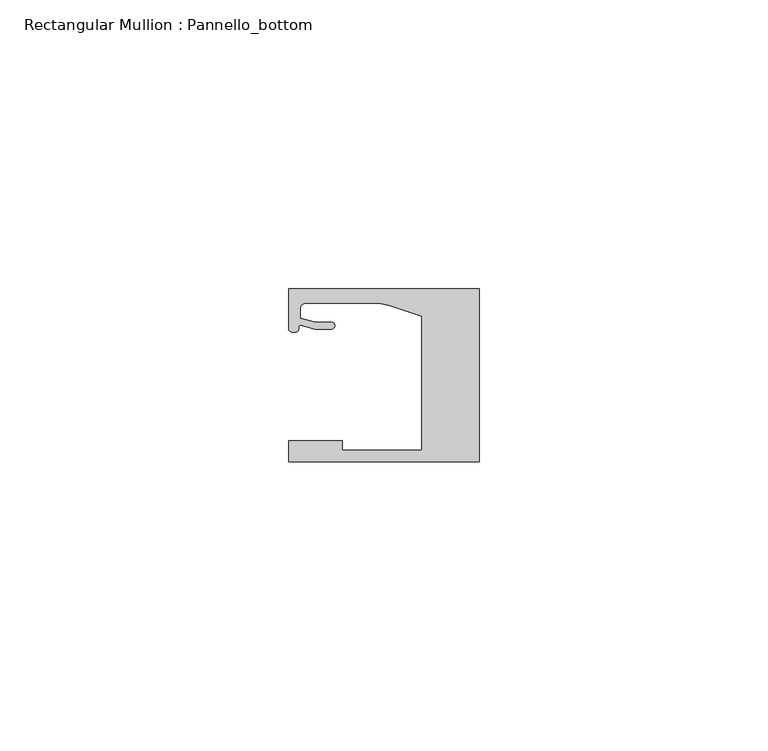
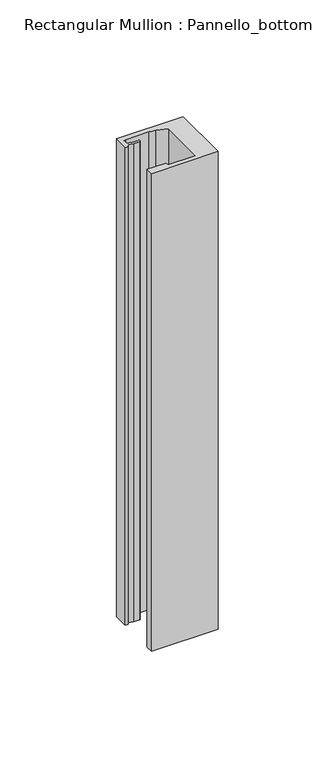
"""IFC4 building model written with IfcOpenShell, lengths in millimetres: member geometry, Rectangular Mullion : Pannello_bottom."""

from ifc_helpers import new_model, si_unit, frame, origin, place, context, project, spatial, polyline, circle_curve, source, transform, mapped, element, save
from ifc_brep_helpers import plane_surface, cylinder_surface, revolved_surface, extruded_surface, spline_curve, advanced_brep


def rectangular_mullion_pannello_bottom_a739c707(model_context):
    return source(origin(), model_context, "Body", "AdvancedBrep", [
        advanced_brep(
        [(-33.0, -15.0, 0.0), (0.0, -15.0, 0.0), (0.0, 15.0, 0.0), (-33.0000135, 15.0, 0.0), (-33.0000135, 8.0000472, 0.0), (-30.9223017, 8.6490241, 0.0), (-28.4999305, 7.9999523, 0.0), (-25.59998, 7.9999523, 0.0), (-25.59998, 9.1999523, 0.0), (-28.3419477, 9.1999523, 0.0), (-31.0, 9.9121746, 0.0), (-31.0, 11.4999419, 0.0), (-30.0000002, 12.4999419, 0.0), (-18.5493024, 12.4999438, 0.0), (-15.4591336, 12.0105099, 0.0), (-9.9999723, 10.2367227, 0.0), (-9.9999723, -13.0000004, 0.0), (-23.700041, -13.0000004, 0.0), (-23.700041, -11.3000004, 0.0), (-33.0, -11.3000004, 0.0), (-33.0, -15.0, -250.0), (-33.0, -11.3000004, -250.0), (-23.700041, -11.3000004, -250.0), (-23.700041, -13.0000004, -250.0), (-9.9999723, -13.0000004, -250.0), (-9.9999723, 10.2367227, -250.0), (-15.4591336, 12.0105099, -250.0), (-18.5493024, 12.4999438, -250.0), (-30.0000002, 12.4999419, -250.0), (-31.0, 11.4999419, -250.0), (-31.0, 9.9121746, -250.0), (-28.3419477, 9.1999523, -250.0), (-25.59998, 9.1999523, -250.0), (-25.59998, 7.9999523, -250.0), (-28.4999305, 7.9999523, -250.0), (-30.9223017, 8.6490241, -250.0), (-33.0000135, 8.0000472, -250.0), (-33.0000135, 15.0, -250.0), (0.0, 15.0, -250.0), (0.0, -15.0, -250.0)],
        [
            (0, 1),
            (1, 2),
            (2, 3),
            (3, 4),
            (4, 5, spline_curve(3, [(-33.0000135, 8.0000472, 0.0), (-33.0000135, 7.457047519, 0.0), (-32.262327879, 7.456527435, 0.0), (-31.357433266, 7.563996614, 0.0), (-31.305645054, 7.690065204, 0.0), (-31.298563602, 8.366228555, 0.0), (-31.312054066, 8.717747958, 0.0), (-30.9223017, 8.6490241, 0.0)], [4, 2, 2, 4], [0.0, 0.0027053965905959043, 0.0058611956533709, 0.007702013405570312])),
            (5, 6),
            (6, 7),
            (7, 8, circle_curve(frame((-25.59998, 8.5999523, 0.0), z_axis=(0.0, 0.0, 1.0), x_axis=(0.0, 1.0, 0.0)), 0.6)),
            (8, 9),
            (9, 10),
            (10, 11),
            (11, 12, circle_curve(frame((-30.0, 11.4999419, 0.0), z_axis=(0.0, 0.0, -1.0), x_axis=(0.0, 1.0, 0.0)), 1.0)),
            (12, 13),
            (13, 14, circle_curve(frame((-18.5493007, 2.4999438, 0.0), z_axis=(0.0, 0.0, -1.0), x_axis=(0.0, 1.0, 0.0)), 10.0)),
            (14, 15),
            (15, 16),
            (16, 17),
            (17, 18),
            (18, 19),
            (19, 0),
            (20, 21),
            (21, 22),
            (22, 23),
            (23, 24),
            (24, 25),
            (25, 26),
            (26, 27, circle_curve(frame((-18.5493007, 2.4999438, -250.0), z_axis=(0.0, 0.0, 1.0), x_axis=(0.0, 1.0, 0.0)), 10.0)),
            (27, 28),
            (28, 29, circle_curve(frame((-30.0, 11.4999419, -250.0), z_axis=(0.0, 0.0, 1.0), x_axis=(0.0, 1.0, 0.0)), 1.0)),
            (29, 30),
            (30, 31),
            (31, 32),
            (32, 33, circle_curve(frame((-25.59998, 8.5999523, -250.0), z_axis=(0.0, 0.0, -1.0), x_axis=(0.0, 1.0, 0.0)), 0.6)),
            (33, 34),
            (34, 35),
            (35, 36, spline_curve(3, [(-30.9223017, 8.6490241, -250.0), (-31.312054066, 8.717747958, -250.0), (-31.298563602, 8.366228555, -250.0), (-31.305645054, 7.690065204, -250.0), (-31.357433266, 7.563996614, -250.0), (-32.262327879, 7.456527435, -250.0), (-33.0000135, 7.457047519, -250.0), (-33.0000135, 8.0000472, -250.0)], [4, 2, 2, 4], [0.0, 0.001840817752199412, 0.004996616814974408, 0.007702013405570312])),
            (36, 37),
            (37, 38),
            (38, 39),
            (39, 20),
            (0, 20),
            (39, 1),
            (38, 2),
            (37, 3),
            (36, 4),
            (35, 5),
            (34, 6),
            (33, 7),
            (32, 8),
            (31, 9),
            (30, 10),
            (29, 11),
            (28, 12),
            (27, 13),
            (26, 14),
            (25, 15),
            (24, 16),
            (23, 17),
            (22, 18),
            (21, 19),
        ],
        [
            plane_surface(frame((0.0, -36.2491502, 0.0), z_axis=(0.0, 0.0, 1.0), x_axis=(-1.0, 0.0, 0.0))),
            plane_surface(frame((0.0, -36.2491502, -250.0), z_axis=(0.0, 0.0, -1.0), x_axis=(-1.0, 0.0, 0.0))),
            plane_surface(frame((-33.0, -15.0, 0.0), z_axis=(0.0, -1.0, 0.0), x_axis=(0.0, 0.0, -1.0))),
            plane_surface(frame((0.0, -15.0, 0.0), z_axis=(1.0, 0.0, 0.0), x_axis=(0.0, 0.0, -1.0))),
            plane_surface(frame((0.0, 15.0, 0.0), z_axis=(0.0, 1.0, 0.0), x_axis=(0.0, 0.0, -1.0))),
            plane_surface(frame((-33.0000135, 15.0, 0.0), z_axis=(-1.0, 0.0, 0.0), x_axis=(0.0, 0.0, -1.0))),
            extruded_surface(spline_curve(3, [(-33.0000135, 8.0000472, -250.0), (-33.0000135, 7.457047519, -250.0), (-32.262327879, 7.456527435, -250.0), (-31.357433266, 7.563996614, -250.0), (-31.305645054, 7.690065204, -250.0), (-31.298563602, 8.366228555, -250.0), (-31.312054066, 8.717747958, -250.0), (-30.9223017, 8.6490241, -250.0)], [4, 2, 2, 4], [0.0, 0.0027053965905959043, 0.0058611956533709, 0.007702013405570312]), (0.0, 0.0, 250.0), 250.0),
            plane_surface(frame((-30.9223017, 8.6490241, 0.0), z_axis=(-0.25881883200192934, -0.9659258833891746, 0.0), x_axis=(0.0, 0.0, -1.0))),
            plane_surface(frame((-28.4999305, 7.9999523, 0.0), z_axis=(0.0, -1.0, 0.0), x_axis=(0.0, 0.0, -1.0))),
            cylinder_surface(frame((-25.59998, 8.5999523, 0.0), z_axis=(0.0, 0.0, 1.0), x_axis=(0.0, 1.0, 0.0)), 0.6),
            plane_surface(frame((-25.59998, 9.1999523, 0.0), z_axis=(0.0, 1.0, 0.0), x_axis=(0.0, 0.0, -1.0))),
            plane_surface(frame((-28.3419477, 9.1999523, 0.0), z_axis=(0.25881883204288636, 0.9659258833782002, 0.0), x_axis=(0.0, 0.0, -1.0))),
            plane_surface(frame((-31.0, 9.9121746, 0.0), z_axis=(1.0, 0.0, 0.0), x_axis=(0.0, 0.0, -1.0))),
            revolved_surface(polyline([(-30.0, 12.4999419, -250.0), (-30.0, 12.4999419, 0.0)]), (-30.0, 11.4999419, 0.0), (0.0, 0.0, -1.0)),
            plane_surface(frame((-30.0000002, 12.4999419, 0.0), z_axis=(1.6923026533778639e-07, -0.9999999999999858, 0.0), x_axis=(0.0, 0.0, -1.0))),
            revolved_surface(polyline([(-18.5493007, 12.4999438, -250.0), (-18.5493007, 12.4999438, 0.0)]), (-18.5493007, 2.4999438, 0.0), (0.0, 0.0, -1.0)),
            plane_surface(frame((-15.4591336, 12.0105099, 0.0), z_axis=(-0.30901670911956314, -0.9510566089801992, 0.0), x_axis=(0.0, 0.0, -1.0))),
            plane_surface(frame((-9.9999723, 10.2367227, 0.0), z_axis=(-1.0, 0.0, 0.0), x_axis=(0.0, 0.0, -1.0))),
            plane_surface(frame((-9.9999723, -13.0000004, 0.0), z_axis=(0.0, 1.0, 0.0), x_axis=(0.0, 0.0, -1.0))),
            plane_surface(frame((-23.700041, -13.0000004, 0.0), z_axis=(1.0, 0.0, 0.0), x_axis=(0.0, 0.0, -1.0))),
            plane_surface(frame((-23.700041, -11.3000004, 0.0), z_axis=(0.0, 1.0, 0.0), x_axis=(0.0, 0.0, -1.0))),
            plane_surface(frame((-33.0, -11.3000004, 0.0), z_axis=(-1.0, 0.0, 0.0), x_axis=(0.0, 0.0, -1.0))),
        ],
        [
            (0, [[1, 2, 3, 4, 5, 6, 7, 8, 9, 10, 11, 12, 13, 14, 15, 16, 17, 18, 19, 20]]),
            (1, [[21, 22, 23, 24, 25, 26, 27, 28, 29, 30, 31, 32, 33, 34, 35, 36, 37, 38, 39, 40]]),
            (2, [[-1, 41, -40, 42]]),
            (3, [[-2, -42, -39, 43]]),
            (4, [[-3, -43, -38, 44]]),
            (5, [[-4, -44, -37, 45]]),
            (6, [[-5, -45, -36, 46]]),
            (7, [[-6, -46, -35, 47]]),
            (8, [[-7, -47, -34, 48]]),
            (9, [[-8, -48, -33, 49]]),
            (10, [[-9, -49, -32, 50]]),
            (11, [[-10, -50, -31, 51]]),
            (12, [[-11, -51, -30, 52]]),
            (13, [[-12, -52, -29, 53]]),
            (14, [[-13, -53, -28, 54]]),
            (15, [[-14, -54, -27, 55]]),
            (16, [[-15, -55, -26, 56]]),
            (17, [[-16, -56, -25, 57]]),
            (18, [[-17, -57, -24, 58]]),
            (19, [[-18, -58, -23, 59]]),
            (20, [[-19, -59, -22, 60]]),
            (21, [[-20, -60, -21, -41]]),
        ],
    ),
    ])


if __name__ == "__main__":
    model = new_model("IFC4")
    model_context = context("Model", 3, world=origin())
    ifc_project = project(units=[si_unit("LENGTHUNIT", "METRE", prefix="MILLI")], contexts=[model_context])
    site = spatial("IfcSite", under=ifc_project)
    building = spatial("IfcBuilding", under=site)
    placement = place(None, origin())
    rectangular_mullion_pannello_bottom_shape = rectangular_mullion_pannello_bottom_a739c707(model_context)
    element("IfcMember", 1, ObjectType="Rectangular Mullion : Pannello_bottom", at=placement, inside=building, context=model_context, shape_type="MappedRepresentation", body=[
        mapped(rectangular_mullion_pannello_bottom_shape, transform((0.0, 0.0, 0.0), x_axis=(1.0, 0.0, 0.0), y_axis=(0.0, 1.0, 0.0), z_axis=(0.0, 0.0, 1.0))),
    ])
    save(model, "model.ifc")

# Revit data of these elements
# Type "Rectangular Mullion : Pannello_bottom"
#   built-in parameter 1007322 = 0.0984252 (stored number, unit not read)
#   built-in parameter 1007321 = 0.0328083 (stored number, unit not read)
#   built-in parameter 1007320 = 0 (stored number, unit not read)
